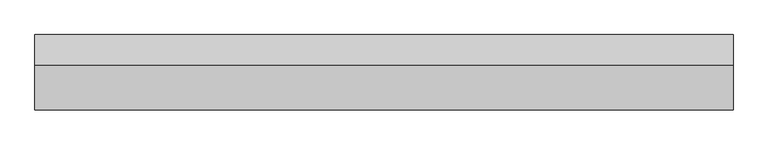
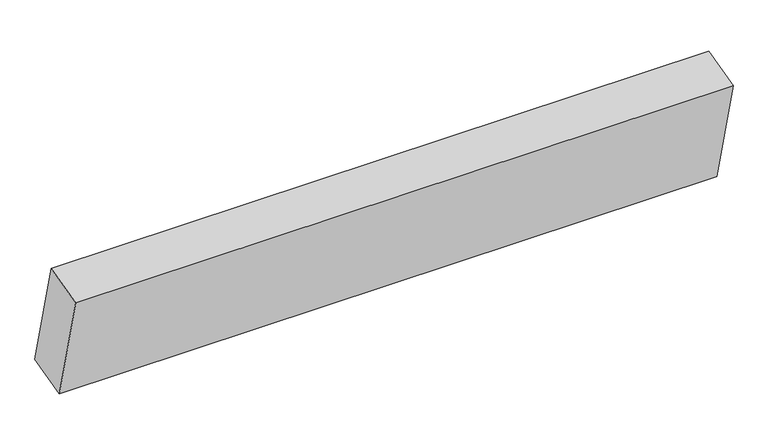
"""IFC4 building model written with IfcOpenShell, lengths in millimetres: proxy geometry, Structure007 595 : Structure007 595."""

import ifcopenshell
import ifcopenshell.guid

model = None  # the IFC model being written
_history = None  # IfcOwnerHistory: only IFC2X3 demands one
_inside = {}  # id of a spatial element -> (the spatial element, [elements in it])
_under = {}  # id of a project, library or spatial element -> (it, [spatial elements below it])
_declared = {}  # id of a project -> (the project, [libraries it declares])
_typed = {}  # id of a type object -> (the type object, [elements of that type])
_made_of = {}  # id of a material, layer set ... -> (it, [elements and type objects made of it])


def new_model(schema):
    """Start an empty IFC model of exactly this schema.

    Asked for "IFC4X3", IfcOpenShell would pick the latest addendum, in which some entities
    have other attributes; the version numbers below select the first issue.
    IFC2X3 requires an IfcOwnerHistory on every rooted entity: one is made here for all.
    """
    global model, _history
    if schema == "IFC4X3":
        model = ifcopenshell.file(schema_version=(4, 3, 0, 0))
    else:
        model = ifcopenshell.file(schema=schema)
    _inside.clear()
    _under.clear()
    _declared.clear()
    _typed.clear()
    _made_of.clear()
    _history = None
    if model.schema == "IFC2X3":
        org = make("IfcOrganization", Name="unknown")
        user = make(
            "IfcPersonAndOrganization",
            ThePerson=make("IfcPerson", FamilyName="unknown"),
            TheOrganization=org,
        )
        app = make(
            "IfcApplication",
            ApplicationDeveloper=org,
            Version="unknown",
            ApplicationFullName="unknown",
            ApplicationIdentifier="unknown",
        )
        _history = make(
            "IfcOwnerHistory",
            OwningUser=user,
            OwningApplication=app,
            ChangeAction="ADDED",
            CreationDate=0,
        )
    return model


def make(cls, **values):
    """One entity of the class cls with the attributes given. An attribute that is None is left unset."""
    return model.create_entity(
        cls, **{name: value for name, value in values.items() if value is not None}
    )


def rooted(cls, **values):
    """An entity with a GlobalId (a new one), such as an element, a storey or a relation."""
    return make(cls, GlobalId=ifcopenshell.guid.new(), OwnerHistory=_history, **values)


def si_unit(unit_type, name, prefix=None):
    """IfcSIUnit, for example si_unit("LENGTHUNIT", "METRE", prefix="MILLI")."""
    return make("IfcSIUnit", UnitType=unit_type, Prefix=prefix, Name=name)


def assignment(units):
    """IfcUnitAssignment: the units of a project."""
    return None if units is None else make("IfcUnitAssignment", Units=units)


def point(xyz):
    """IfcCartesianPoint."""
    return None if xyz is None else make("IfcCartesianPoint", Coordinates=xyz)


def direction(xyz):
    """IfcDirection."""
    return None if xyz is None else make("IfcDirection", DirectionRatios=xyz)


def frame(location, z_axis=None, x_axis=None):
    """IfcAxis2Placement3D, a coordinate frame: its origin and axes. An axis left out is left unset."""
    return make(
        "IfcAxis2Placement3D",
        Location=point(location),
        Axis=direction(z_axis),
        RefDirection=direction(x_axis),
    )


def origin():
    """The frame at (0, 0, 0) with its axes left unset."""
    return frame((0.0, 0.0, 0.0))


def place(relative_to, where):
    """IfcLocalPlacement: puts the frame where relative to a parent placement (None: the world)."""
    return make(
        "IfcLocalPlacement", PlacementRelTo=relative_to, RelativePlacement=where
    )


def context(
    kind, dimensions, precision=None, world=None, true_north=None, identifier=None
):
    """IfcGeometricRepresentationContext, for example the 3D "Model" context."""
    return make(
        "IfcGeometricRepresentationContext",
        ContextIdentifier=identifier,
        ContextType=kind,
        CoordinateSpaceDimension=dimensions,
        Precision=precision,
        WorldCoordinateSystem=world,
        TrueNorth=true_north,
    )


def project(units=None, contexts=None):
    """IfcProject with its units and contexts."""
    return rooted(
        "IfcProject",
        Name="project",
        RepresentationContexts=contexts,
        UnitsInContext=assignment(units),
    )


def spatial(cls, under=None, at=None, **own):
    """A site, building, storey or space (cls), placed at a placement, below another one or the project."""
    s = rooted(cls, ObjectPlacement=at, **own)
    if under is not None:
        _under.setdefault(under.id(), (under, []))[1].append(s)
    return s


def polyline(points):
    """IfcPolyline through the points."""
    return make("IfcPolyline", Points=[point(p) for p in points])


def outline(outer, holes=None, kind="AREA"):
    """IfcArbitraryClosedProfileDef: a profile drawn as a closed curve; with holes, ...WithVoids."""
    if holes is None:
        return make("IfcArbitraryClosedProfileDef", ProfileType=kind, OuterCurve=outer)
    return make(
        "IfcArbitraryProfileDefWithVoids",
        ProfileType=kind,
        OuterCurve=outer,
        InnerCurves=holes,
    )


def extrude(swept, where, along, depth):
    """IfcExtrudedAreaSolid: the profile swept, set in the frame where, extruded along a direction by depth."""
    return make(
        "IfcExtrudedAreaSolid",
        SweptArea=swept,
        Position=where,
        ExtrudedDirection=direction(along),
        Depth=depth,
    )


def shape(context_of_items, identifier, shape_type, items):
    """IfcShapeRepresentation: the items that make up one representation, for example the "Body"."""
    return make(
        "IfcShapeRepresentation",
        ContextOfItems=context_of_items,
        RepresentationIdentifier=identifier,
        RepresentationType=shape_type,
        Items=items,
    )


def source(mapping_origin, context_of_items, identifier, shape_type, items):
    """IfcRepresentationMap: a shape defined once, which mapped items show again and again."""
    return make(
        "IfcRepresentationMap",
        MappingOrigin=mapping_origin,
        MappedRepresentation=shape(context_of_items, identifier, shape_type, items),
    )


def transform(
    local_origin,
    x_axis=None,
    y_axis=None,
    z_axis=None,
    scale=None,
    scale2=None,
    scale3=None,
    uniform=True,
):
    """IfcCartesianTransformationOperator3D, or its non-uniform kind. x_axis, y_axis, z_axis: its Axis1, 2, 3."""
    if uniform:
        return make(
            "IfcCartesianTransformationOperator3D",
            Axis1=direction(x_axis),
            Axis2=direction(y_axis),
            LocalOrigin=point(local_origin),
            Scale=scale,
            Axis3=direction(z_axis),
        )
    return make(
        "IfcCartesianTransformationOperator3DnonUniform",
        Axis1=direction(x_axis),
        Axis2=direction(y_axis),
        LocalOrigin=point(local_origin),
        Scale=scale,
        Axis3=direction(z_axis),
        Scale2=scale2,
        Scale3=scale3,
    )


def mapped(mapping_source, mapping_target):
    """IfcMappedItem: shows the shape of a source again, moved by a transform."""
    return make(
        "IfcMappedItem", MappingSource=mapping_source, MappingTarget=mapping_target
    )


def made_of(thing, what):
    """Note that an element or type object is made of a material, layer set ...; save() writes the relation."""
    if what is not None:
        _made_of.setdefault(what.id(), (what, []))[1].append(thing)
    return thing


def element(
    cls,
    number,
    at=None,
    inside=None,
    cuts=None,
    type_object=None,
    material=None,
    context=None,
    identifier="Body",
    shape_type=None,
    held_by="IfcProductDefinitionShape",
    body=None,
    shapes=None,
    **own,
):
    """One element of the class cls, such as IfcWall. Its Tag is "e" and its number.

    at: its placement. inside: the storey or other place that contains it. cuts: it is an
    opening in that element (IfcRelVoidsElement). A single representation is given by context,
    identifier, shape_type and body (its items); several are given by shapes. held_by: the class
    of the entity that holds the representations. save() writes the other relations.
    """
    e = rooted(cls, Tag="e%d" % number, ObjectPlacement=at, **own)
    if body is not None:
        shapes = [shape(context, identifier, shape_type, body)]
    if shapes is not None:
        e.Representation = make(held_by, Representations=shapes)
    if inside is not None:
        _inside.setdefault(inside.id(), (inside, []))[1].append(e)
    if cuts is not None:
        rooted(
            "IfcRelVoidsElement", RelatingBuildingElement=cuts, RelatedOpeningElement=e
        )
    if type_object is not None:
        _typed.setdefault(type_object.id(), (type_object, []))[1].append(e)
    return made_of(e, material)


def aggregate(whole, parts):
    """IfcRelAggregates: a whole, such as a stair, and the parts it consists of."""
    return rooted("IfcRelAggregates", RelatingObject=whole, RelatedObjects=parts)


def save(model, path):
    """Write the relations noted so far, then the file.

    IfcRelAggregates (storeys below a building ...), IfcRelContainedInSpatialStructure (elements
    in a storey), IfcRelDefinesByType, IfcRelAssociatesMaterial and IfcRelDeclares: one each for
    every whole, place, type object, material and project.
    """
    for whole, parts in _under.values():
        aggregate(whole, parts)
    for where, things in _inside.values():
        rooted(
            "IfcRelContainedInSpatialStructure",
            RelatedElements=things,
            RelatingStructure=where,
        )
    for kind, things in _typed.values():
        rooted("IfcRelDefinesByType", RelatedObjects=things, RelatingType=kind)
    for what, things in _made_of.values():
        rooted("IfcRelAssociatesMaterial", RelatedObjects=things, RelatingMaterial=what)
    for by, libraries in _declared.values():
        rooted("IfcRelDeclares", RelatingContext=by, RelatedDefinitions=libraries)
    model.write(path)


def generic_models_ce666b17(model_context):
    return source(origin(), model_context, "Body", "SweptSolid", [
        extrude(outline(polyline([(0.0, -133.35), (0.0, 0.0), (2000.0, 0.0), (2000.0, -133.35), (0.0, -133.35)])), frame((3694.2883192, 9633.2576598, 43211.937945), z_axis=(0.0, -0.2425992307954678, 0.9701265964900908), x_axis=(1.0, 0.0, 0.0)), (0.0, 0.0, 1.0), 355.6),
    ])


if __name__ == "__main__":
    model = new_model("IFC4")
    model_context = context("Model", 3, world=origin())
    ifc_project = project(units=[si_unit("LENGTHUNIT", "METRE", prefix="MILLI")], contexts=[model_context])
    site = spatial("IfcSite", under=ifc_project)
    building = spatial("IfcBuilding", under=site)
    placement = place(None, origin())
    generic_models_shape = generic_models_ce666b17(model_context)
    element("IfcBuildingElementProxy", 1, Name="Structure007 595 : Structure007 595", ObjectType="Structure007 595 : Structure007 595", at=placement, inside=building, context=model_context, shape_type="MappedRepresentation", body=[
        mapped(generic_models_shape, transform((0.0, 0.0, 0.0), x_axis=(1.0, 0.0, 0.0), y_axis=(0.0, 1.0, 0.0), z_axis=(0.0, 0.0, 1.0))),
    ])
    save(model, "model.ifc")

# Revit data of these elements
# Type "Structure007 595 : Structure007 595"
#   NameOverride = "Structure007"
# Element 1 (IfcBuildingElementProxy, "Structure007 595 : Structure007 595")
#   Materials on its faces: "STRUCTURAL MEMBER (SEE STRUCTURAL DWGS)"
# Materials
#   "STRUCTURAL MEMBER (SEE STRUCTURAL DWGS)": class "Unassigned", colour RGB 176 134 95, transparency 0, Cost = 0
